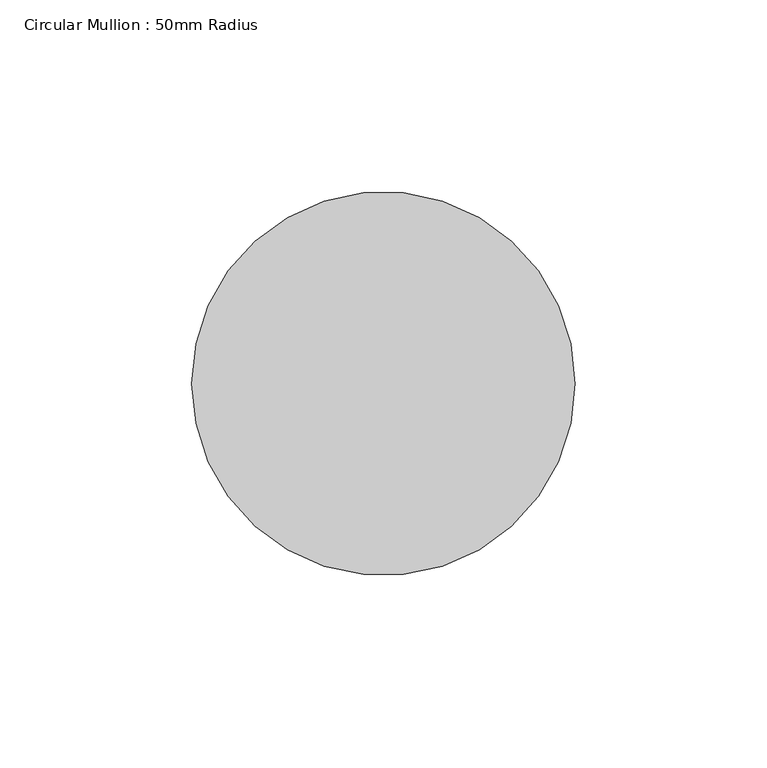
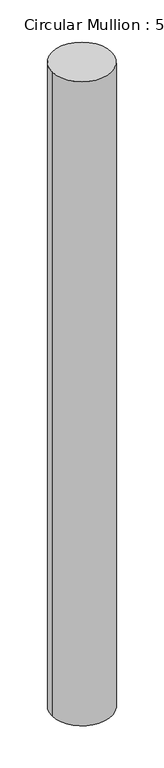
"""IFC4 building model written with IfcOpenShell, lengths in millimetres: member geometry, Circular Mullion : 50mm Radius."""

from ifc_helpers import new_model, si_unit, point, frame, origin, origin_2d, place, context, project, spatial, circle_curve, trimmed, segment, composite_curve, outline, extrude, source, transform, mapped, element, save


def circular_mullion_50mm_radius_cba37685(model_context):
    return source(origin(), model_context, "Body", "SweptSolid", [
        extrude(outline(composite_curve([segment(trimmed(circle_curve(origin_2d(), 50.0), [point((50.0, 0.0))], [point((-50.0, 0.0))], False, "CARTESIAN"), True, "CONTINUOUS"), segment(trimmed(circle_curve(origin_2d(), 50.0), [point((-50.0, 0.0))], [point((50.0, 0.0))], False, "CARTESIAN"), True, "CONTINUOUS")], self_intersect=False)), frame((0.0, 0.0, -1138.7077787), z_axis=(0.0, 0.0, 1.0), x_axis=(1.0, 0.0, 0.0)), (0.0, 0.0, 1.0), 1138.7077787),
    ])


if __name__ == "__main__":
    model = new_model("IFC4")
    model_context = context("Model", 3, world=origin())
    ifc_project = project(units=[si_unit("LENGTHUNIT", "METRE", prefix="MILLI")], contexts=[model_context])
    site = spatial("IfcSite", under=ifc_project)
    building = spatial("IfcBuilding", under=site)
    placement = place(None, origin())
    circular_mullion_50mm_radius_shape = circular_mullion_50mm_radius_cba37685(model_context)
    element("IfcMember", 1, ObjectType="Circular Mullion : 50mm Radius", at=placement, inside=building, context=model_context, shape_type="MappedRepresentation", body=[
        mapped(circular_mullion_50mm_radius_shape, transform((0.0, 0.0, 0.0), x_axis=(1.0, 0.0, 0.0), y_axis=(0.0, 1.0, 0.0), z_axis=(0.0, 0.0, 1.0))),
    ])
    save(model, "model.ifc")

# Revit data of these elements
# Type "Circular Mullion : 50mm Radius"
#   built-in parameter 1007350 = 0.164042 (stored number, unit not read)
# Element 1 (IfcMember, "Circular Mullion : 50mm Radius")
#   Materials on its faces: "Aluminium"
# Materials
#   "Aluminium": class "Metal", colour RGB 247 247 247, transparency 0, Description = "Aluminium 6061", Cost = 0
